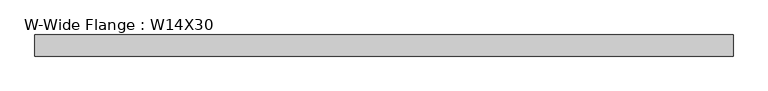
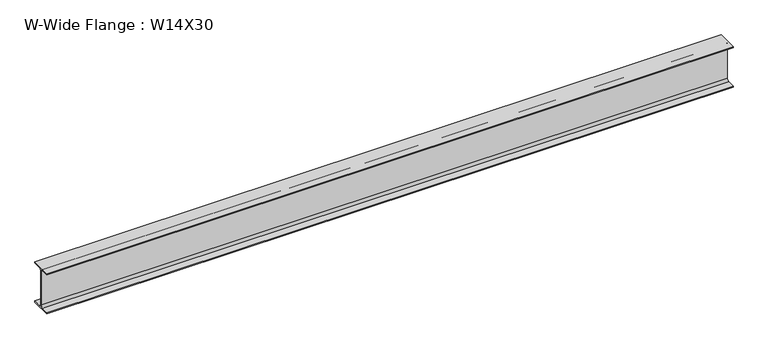
"""IFC4 building model written with IfcOpenShell, lengths in millimetres: beam geometry, W-Wide Flange : W14X30."""

import ifcopenshell
import ifcopenshell.guid

model = None  # the IFC model being written
_history = None  # IfcOwnerHistory: only IFC2X3 demands one
_inside = {}  # id of a spatial element -> (the spatial element, [elements in it])
_under = {}  # id of a project, library or spatial element -> (it, [spatial elements below it])
_declared = {}  # id of a project -> (the project, [libraries it declares])
_typed = {}  # id of a type object -> (the type object, [elements of that type])
_made_of = {}  # id of a material, layer set ... -> (it, [elements and type objects made of it])


def new_model(schema):
    """Start an empty IFC model of exactly this schema.

    Asked for "IFC4X3", IfcOpenShell would pick the latest addendum, in which some entities
    have other attributes; the version numbers below select the first issue.
    IFC2X3 requires an IfcOwnerHistory on every rooted entity: one is made here for all.
    """
    global model, _history
    if schema == "IFC4X3":
        model = ifcopenshell.file(schema_version=(4, 3, 0, 0))
    else:
        model = ifcopenshell.file(schema=schema)
    _inside.clear()
    _under.clear()
    _declared.clear()
    _typed.clear()
    _made_of.clear()
    _history = None
    if model.schema == "IFC2X3":
        org = make("IfcOrganization", Name="unknown")
        user = make(
            "IfcPersonAndOrganization",
            ThePerson=make("IfcPerson", FamilyName="unknown"),
            TheOrganization=org,
        )
        app = make(
            "IfcApplication",
            ApplicationDeveloper=org,
            Version="unknown",
            ApplicationFullName="unknown",
            ApplicationIdentifier="unknown",
        )
        _history = make(
            "IfcOwnerHistory",
            OwningUser=user,
            OwningApplication=app,
            ChangeAction="ADDED",
            CreationDate=0,
        )
    return model


def make(cls, **values):
    """One entity of the class cls with the attributes given. An attribute that is None is left unset."""
    return model.create_entity(
        cls, **{name: value for name, value in values.items() if value is not None}
    )


def rooted(cls, **values):
    """An entity with a GlobalId (a new one), such as an element, a storey or a relation."""
    return make(cls, GlobalId=ifcopenshell.guid.new(), OwnerHistory=_history, **values)


def si_unit(unit_type, name, prefix=None):
    """IfcSIUnit, for example si_unit("LENGTHUNIT", "METRE", prefix="MILLI")."""
    return make("IfcSIUnit", UnitType=unit_type, Prefix=prefix, Name=name)


def assignment(units):
    """IfcUnitAssignment: the units of a project."""
    return None if units is None else make("IfcUnitAssignment", Units=units)


def point(xyz):
    """IfcCartesianPoint."""
    return None if xyz is None else make("IfcCartesianPoint", Coordinates=xyz)


def direction(xyz):
    """IfcDirection."""
    return None if xyz is None else make("IfcDirection", DirectionRatios=xyz)


def frame(location, z_axis=None, x_axis=None):
    """IfcAxis2Placement3D, a coordinate frame: its origin and axes. An axis left out is left unset."""
    return make(
        "IfcAxis2Placement3D",
        Location=point(location),
        Axis=direction(z_axis),
        RefDirection=direction(x_axis),
    )


def frame_2d(location, x_axis=None):
    """IfcAxis2Placement2D, a coordinate frame in the plane: its origin and x axis."""
    return make(
        "IfcAxis2Placement2D", Location=point(location), RefDirection=direction(x_axis)
    )


def origin():
    """The frame at (0, 0, 0) with its axes left unset."""
    return frame((0.0, 0.0, 0.0))


def place(relative_to, where):
    """IfcLocalPlacement: puts the frame where relative to a parent placement (None: the world)."""
    return make(
        "IfcLocalPlacement", PlacementRelTo=relative_to, RelativePlacement=where
    )


def context(
    kind, dimensions, precision=None, world=None, true_north=None, identifier=None
):
    """IfcGeometricRepresentationContext, for example the 3D "Model" context."""
    return make(
        "IfcGeometricRepresentationContext",
        ContextIdentifier=identifier,
        ContextType=kind,
        CoordinateSpaceDimension=dimensions,
        Precision=precision,
        WorldCoordinateSystem=world,
        TrueNorth=true_north,
    )


def project(units=None, contexts=None):
    """IfcProject with its units and contexts."""
    return rooted(
        "IfcProject",
        Name="project",
        RepresentationContexts=contexts,
        UnitsInContext=assignment(units),
    )


def spatial(cls, under=None, at=None, **own):
    """A site, building, storey or space (cls), placed at a placement, below another one or the project."""
    s = rooted(cls, ObjectPlacement=at, **own)
    if under is not None:
        _under.setdefault(under.id(), (under, []))[1].append(s)
    return s


def polyline(points):
    """IfcPolyline through the points."""
    return make("IfcPolyline", Points=[point(p) for p in points])


def circle_curve(where, radius):
    """IfcCircle in the frame where."""
    return make("IfcCircle", Position=where, Radius=radius)


def trimmed(basis, trim1, trim2, sense, master):
    """IfcTrimmedCurve: the piece of a basis curve between two trims."""
    return make(
        "IfcTrimmedCurve",
        BasisCurve=basis,
        Trim1=trim1,
        Trim2=trim2,
        SenseAgreement=sense,
        MasterRepresentation=master,
    )


def segment(curve, same_sense, transition):
    """IfcCompositeCurveSegment."""
    return make(
        "IfcCompositeCurveSegment",
        Transition=transition,
        SameSense=same_sense,
        ParentCurve=curve,
    )


def composite_curve(segments, self_intersect=None):
    """IfcCompositeCurve: segments joined end to end."""
    return make("IfcCompositeCurve", Segments=segments, SelfIntersect=self_intersect)


def outline(outer, holes=None, kind="AREA"):
    """IfcArbitraryClosedProfileDef: a profile drawn as a closed curve; with holes, ...WithVoids."""
    if holes is None:
        return make("IfcArbitraryClosedProfileDef", ProfileType=kind, OuterCurve=outer)
    return make(
        "IfcArbitraryProfileDefWithVoids",
        ProfileType=kind,
        OuterCurve=outer,
        InnerCurves=holes,
    )


def extrude(swept, where, along, depth):
    """IfcExtrudedAreaSolid: the profile swept, set in the frame where, extruded along a direction by depth."""
    return make(
        "IfcExtrudedAreaSolid",
        SweptArea=swept,
        Position=where,
        ExtrudedDirection=direction(along),
        Depth=depth,
    )


def shape(context_of_items, identifier, shape_type, items):
    """IfcShapeRepresentation: the items that make up one representation, for example the "Body"."""
    return make(
        "IfcShapeRepresentation",
        ContextOfItems=context_of_items,
        RepresentationIdentifier=identifier,
        RepresentationType=shape_type,
        Items=items,
    )


def source(mapping_origin, context_of_items, identifier, shape_type, items):
    """IfcRepresentationMap: a shape defined once, which mapped items show again and again."""
    return make(
        "IfcRepresentationMap",
        MappingOrigin=mapping_origin,
        MappedRepresentation=shape(context_of_items, identifier, shape_type, items),
    )


def transform(
    local_origin,
    x_axis=None,
    y_axis=None,
    z_axis=None,
    scale=None,
    scale2=None,
    scale3=None,
    uniform=True,
):
    """IfcCartesianTransformationOperator3D, or its non-uniform kind. x_axis, y_axis, z_axis: its Axis1, 2, 3."""
    if uniform:
        return make(
            "IfcCartesianTransformationOperator3D",
            Axis1=direction(x_axis),
            Axis2=direction(y_axis),
            LocalOrigin=point(local_origin),
            Scale=scale,
            Axis3=direction(z_axis),
        )
    return make(
        "IfcCartesianTransformationOperator3DnonUniform",
        Axis1=direction(x_axis),
        Axis2=direction(y_axis),
        LocalOrigin=point(local_origin),
        Scale=scale,
        Axis3=direction(z_axis),
        Scale2=scale2,
        Scale3=scale3,
    )


def mapped(mapping_source, mapping_target):
    """IfcMappedItem: shows the shape of a source again, moved by a transform."""
    return make(
        "IfcMappedItem", MappingSource=mapping_source, MappingTarget=mapping_target
    )


def made_of(thing, what):
    """Note that an element or type object is made of a material, layer set ...; save() writes the relation."""
    if what is not None:
        _made_of.setdefault(what.id(), (what, []))[1].append(thing)
    return thing


def element(
    cls,
    number,
    at=None,
    inside=None,
    cuts=None,
    type_object=None,
    material=None,
    context=None,
    identifier="Body",
    shape_type=None,
    held_by="IfcProductDefinitionShape",
    body=None,
    shapes=None,
    **own,
):
    """One element of the class cls, such as IfcWall. Its Tag is "e" and its number.

    at: its placement. inside: the storey or other place that contains it. cuts: it is an
    opening in that element (IfcRelVoidsElement). A single representation is given by context,
    identifier, shape_type and body (its items); several are given by shapes. held_by: the class
    of the entity that holds the representations. save() writes the other relations.
    """
    e = rooted(cls, Tag="e%d" % number, ObjectPlacement=at, **own)
    if body is not None:
        shapes = [shape(context, identifier, shape_type, body)]
    if shapes is not None:
        e.Representation = make(held_by, Representations=shapes)
    if inside is not None:
        _inside.setdefault(inside.id(), (inside, []))[1].append(e)
    if cuts is not None:
        rooted(
            "IfcRelVoidsElement", RelatingBuildingElement=cuts, RelatedOpeningElement=e
        )
    if type_object is not None:
        _typed.setdefault(type_object.id(), (type_object, []))[1].append(e)
    return made_of(e, material)


def aggregate(whole, parts):
    """IfcRelAggregates: a whole, such as a stair, and the parts it consists of."""
    return rooted("IfcRelAggregates", RelatingObject=whole, RelatedObjects=parts)


def save(model, path):
    """Write the relations noted so far, then the file.

    IfcRelAggregates (storeys below a building ...), IfcRelContainedInSpatialStructure (elements
    in a storey), IfcRelDefinesByType, IfcRelAssociatesMaterial and IfcRelDeclares: one each for
    every whole, place, type object, material and project.
    """
    for whole, parts in _under.values():
        aggregate(whole, parts)
    for where, things in _inside.values():
        rooted(
            "IfcRelContainedInSpatialStructure",
            RelatedElements=things,
            RelatingStructure=where,
        )
    for kind, things in _typed.values():
        rooted("IfcRelDefinesByType", RelatedObjects=things, RelatingType=kind)
    for what, things in _made_of.values():
        rooted("IfcRelAssociatesMaterial", RelatedObjects=things, RelatingMaterial=what)
    for by, libraries in _declared.values():
        rooted("IfcRelDeclares", RelatingContext=by, RelatedDefinitions=libraries)
    model.write(path)


def w_wide_flange_w14x30_e86b3798(model_context):
    return source(origin(), model_context, "Body", "SweptSolid", [
        extrude(outline(composite_curve([segment(polyline([(85.4769531, -165.9433594), (85.4769531, -175.7660156), (-85.4769531, -175.7660156), (-85.4769531, -165.9433594), (-22.1753906, -165.9433594)]), True, "CONTINUOUS"), segment(trimmed(circle_curve(frame_2d((-22.1753906, -147.1910156)), 18.7523438), [point((-22.1753906, -165.9433594))], [point((-3.4230469, -147.1910156))], True, "CARTESIAN"), True, "CONTINUOUS"), segment(polyline([(-3.4230469, -147.1910156), (-3.4230469, 147.1910156)]), True, "CONTINUOUS"), segment(trimmed(circle_curve(frame_2d((-22.1753906, 147.1910156)), 18.7523438), [point((-3.4230469, 147.1910156))], [point((-22.1753906, 165.9433594))], True, "CARTESIAN"), True, "CONTINUOUS"), segment(polyline([(-22.1753906, 165.9433594), (-85.4769531, 165.9433594), (-85.4769531, 175.7660156), (85.4769531, 175.7660156), (85.4769531, 165.9433594), (22.1753906, 165.9433594)]), True, "CONTINUOUS"), segment(trimmed(circle_curve(frame_2d((22.1753906, 147.1910156)), 18.7523438), [point((22.1753906, 165.9433594))], [point((3.4230469, 147.1910156))], True, "CARTESIAN"), True, "CONTINUOUS"), segment(polyline([(3.4230469, 147.1910156), (3.4230469, -147.1910156)]), True, "CONTINUOUS"), segment(trimmed(circle_curve(frame_2d((22.1753906, -147.1910156)), 18.7523438), [point((3.4230469, -147.1910156))], [point((22.1753906, -165.9433594))], True, "CARTESIAN"), True, "CONTINUOUS"), segment(polyline([(22.1753906, -165.9433594), (85.4769531, -165.9433594)]), True, "CONTINUOUS")], self_intersect=False)), frame((-2801.6835, 0.0, 0.0), z_axis=(1.0, 0.0, 0.0), x_axis=(0.0, 1.0, 0.0)), (0.0, 0.0, 1.0), 5651.246),
    ])


if __name__ == "__main__":
    model = new_model("IFC4")
    model_context = context("Model", 3, world=origin())
    ifc_project = project(units=[si_unit("LENGTHUNIT", "METRE", prefix="MILLI")], contexts=[model_context])
    site = spatial("IfcSite", under=ifc_project)
    building = spatial("IfcBuilding", under=site)
    placement = place(None, origin())
    w_wide_flange_w14x30_shape = w_wide_flange_w14x30_e86b3798(model_context)
    element("IfcBeam", 1, ObjectType="W-Wide Flange : W14X30", at=placement, inside=building, context=model_context, shape_type="MappedRepresentation", body=[
        mapped(w_wide_flange_w14x30_shape, transform((0.0, 0.0, 0.0), x_axis=(1.0, 0.0, 0.0), y_axis=(0.0, 1.0, 0.0), z_axis=(0.0, 0.0, 1.0))),
    ])
    save(model, "model.ifc")

# Revit data of these elements
# Type "W-Wide Flange : W14X30"
#   Assembly Code = "B10"
#   W = 30
#   Length [instance default] = 1524 mm
#   bf = 170.954 mm
#   d = 351.532 mm
#   k = 28.575 mm
#   k2 = 18.752 mm
#   tf = 9.823 mm
#   tw = 6.846 mm
#   A = 0.00557418 m²
#   Structural Material [instance default] = Steel ASTM A992
# Element 1 (IfcBeam, "W-Wide Flange : W14X30")
#   Structural Material = Aluminum, Anodized Red
#   Materials on its faces: "Aluminum, Anodized Red"
# Materials
#   "Steel ASTM A992": class "Metal", colour RGB 128 0 0, transparency 0, Description = "Structural steel 50ksi", Cost = 0
#   "Aluminum, Anodized Red": class "Metal", colour RGB 120 120 120, transparency 0, Description = "Anodized aluminum, red", Cost = 0
